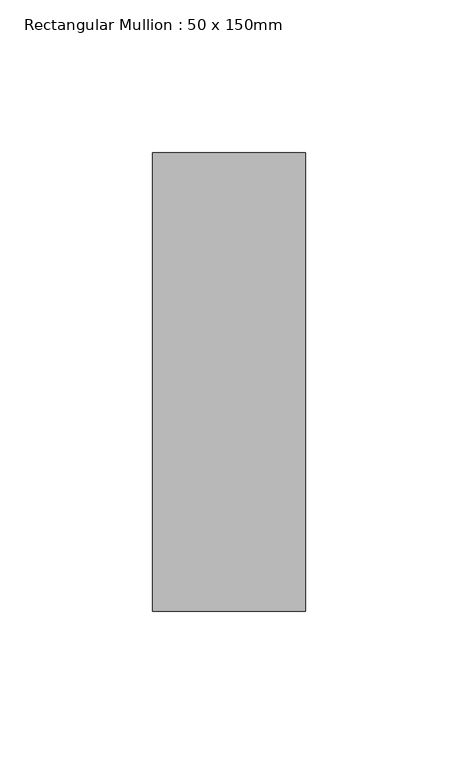
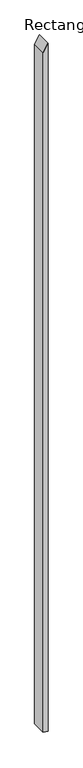
"""IFC4 building model written with IfcOpenShell, lengths in millimetres: member geometry, Rectangular Mullion : 50 x 150mm."""

import ifcopenshell
import ifcopenshell.guid

model = None  # the IFC model being written
_history = None  # IfcOwnerHistory: only IFC2X3 demands one
_inside = {}  # id of a spatial element -> (the spatial element, [elements in it])
_under = {}  # id of a project, library or spatial element -> (it, [spatial elements below it])
_declared = {}  # id of a project -> (the project, [libraries it declares])
_typed = {}  # id of a type object -> (the type object, [elements of that type])
_made_of = {}  # id of a material, layer set ... -> (it, [elements and type objects made of it])


def new_model(schema):
    """Start an empty IFC model of exactly this schema.

    Asked for "IFC4X3", IfcOpenShell would pick the latest addendum, in which some entities
    have other attributes; the version numbers below select the first issue.
    IFC2X3 requires an IfcOwnerHistory on every rooted entity: one is made here for all.
    """
    global model, _history
    if schema == "IFC4X3":
        model = ifcopenshell.file(schema_version=(4, 3, 0, 0))
    else:
        model = ifcopenshell.file(schema=schema)
    _inside.clear()
    _under.clear()
    _declared.clear()
    _typed.clear()
    _made_of.clear()
    _history = None
    if model.schema == "IFC2X3":
        org = make("IfcOrganization", Name="unknown")
        user = make(
            "IfcPersonAndOrganization",
            ThePerson=make("IfcPerson", FamilyName="unknown"),
            TheOrganization=org,
        )
        app = make(
            "IfcApplication",
            ApplicationDeveloper=org,
            Version="unknown",
            ApplicationFullName="unknown",
            ApplicationIdentifier="unknown",
        )
        _history = make(
            "IfcOwnerHistory",
            OwningUser=user,
            OwningApplication=app,
            ChangeAction="ADDED",
            CreationDate=0,
        )
    return model


def make(cls, **values):
    """One entity of the class cls with the attributes given. An attribute that is None is left unset."""
    return model.create_entity(
        cls, **{name: value for name, value in values.items() if value is not None}
    )


def rooted(cls, **values):
    """An entity with a GlobalId (a new one), such as an element, a storey or a relation."""
    return make(cls, GlobalId=ifcopenshell.guid.new(), OwnerHistory=_history, **values)


def si_unit(unit_type, name, prefix=None):
    """IfcSIUnit, for example si_unit("LENGTHUNIT", "METRE", prefix="MILLI")."""
    return make("IfcSIUnit", UnitType=unit_type, Prefix=prefix, Name=name)


def assignment(units):
    """IfcUnitAssignment: the units of a project."""
    return None if units is None else make("IfcUnitAssignment", Units=units)


def point(xyz):
    """IfcCartesianPoint."""
    return None if xyz is None else make("IfcCartesianPoint", Coordinates=xyz)


def direction(xyz):
    """IfcDirection."""
    return None if xyz is None else make("IfcDirection", DirectionRatios=xyz)


def frame(location, z_axis=None, x_axis=None):
    """IfcAxis2Placement3D, a coordinate frame: its origin and axes. An axis left out is left unset."""
    return make(
        "IfcAxis2Placement3D",
        Location=point(location),
        Axis=direction(z_axis),
        RefDirection=direction(x_axis),
    )


def origin():
    """The frame at (0, 0, 0) with its axes left unset."""
    return frame((0.0, 0.0, 0.0))


def place(relative_to, where):
    """IfcLocalPlacement: puts the frame where relative to a parent placement (None: the world)."""
    return make(
        "IfcLocalPlacement", PlacementRelTo=relative_to, RelativePlacement=where
    )


def context(
    kind, dimensions, precision=None, world=None, true_north=None, identifier=None
):
    """IfcGeometricRepresentationContext, for example the 3D "Model" context."""
    return make(
        "IfcGeometricRepresentationContext",
        ContextIdentifier=identifier,
        ContextType=kind,
        CoordinateSpaceDimension=dimensions,
        Precision=precision,
        WorldCoordinateSystem=world,
        TrueNorth=true_north,
    )


def project(units=None, contexts=None):
    """IfcProject with its units and contexts."""
    return rooted(
        "IfcProject",
        Name="project",
        RepresentationContexts=contexts,
        UnitsInContext=assignment(units),
    )


def spatial(cls, under=None, at=None, **own):
    """A site, building, storey or space (cls), placed at a placement, below another one or the project."""
    s = rooted(cls, ObjectPlacement=at, **own)
    if under is not None:
        _under.setdefault(under.id(), (under, []))[1].append(s)
    return s


def polyline(points):
    """IfcPolyline through the points."""
    return make("IfcPolyline", Points=[point(p) for p in points])


def outline(outer, holes=None, kind="AREA"):
    """IfcArbitraryClosedProfileDef: a profile drawn as a closed curve; with holes, ...WithVoids."""
    if holes is None:
        return make("IfcArbitraryClosedProfileDef", ProfileType=kind, OuterCurve=outer)
    return make(
        "IfcArbitraryProfileDefWithVoids",
        ProfileType=kind,
        OuterCurve=outer,
        InnerCurves=holes,
    )


def extrude(swept, where, along, depth):
    """IfcExtrudedAreaSolid: the profile swept, set in the frame where, extruded along a direction by depth."""
    return make(
        "IfcExtrudedAreaSolid",
        SweptArea=swept,
        Position=where,
        ExtrudedDirection=direction(along),
        Depth=depth,
    )


def shape(context_of_items, identifier, shape_type, items):
    """IfcShapeRepresentation: the items that make up one representation, for example the "Body"."""
    return make(
        "IfcShapeRepresentation",
        ContextOfItems=context_of_items,
        RepresentationIdentifier=identifier,
        RepresentationType=shape_type,
        Items=items,
    )


def source(mapping_origin, context_of_items, identifier, shape_type, items):
    """IfcRepresentationMap: a shape defined once, which mapped items show again and again."""
    return make(
        "IfcRepresentationMap",
        MappingOrigin=mapping_origin,
        MappedRepresentation=shape(context_of_items, identifier, shape_type, items),
    )


def transform(
    local_origin,
    x_axis=None,
    y_axis=None,
    z_axis=None,
    scale=None,
    scale2=None,
    scale3=None,
    uniform=True,
):
    """IfcCartesianTransformationOperator3D, or its non-uniform kind. x_axis, y_axis, z_axis: its Axis1, 2, 3."""
    if uniform:
        return make(
            "IfcCartesianTransformationOperator3D",
            Axis1=direction(x_axis),
            Axis2=direction(y_axis),
            LocalOrigin=point(local_origin),
            Scale=scale,
            Axis3=direction(z_axis),
        )
    return make(
        "IfcCartesianTransformationOperator3DnonUniform",
        Axis1=direction(x_axis),
        Axis2=direction(y_axis),
        LocalOrigin=point(local_origin),
        Scale=scale,
        Axis3=direction(z_axis),
        Scale2=scale2,
        Scale3=scale3,
    )


def mapped(mapping_source, mapping_target):
    """IfcMappedItem: shows the shape of a source again, moved by a transform."""
    return make(
        "IfcMappedItem", MappingSource=mapping_source, MappingTarget=mapping_target
    )


def made_of(thing, what):
    """Note that an element or type object is made of a material, layer set ...; save() writes the relation."""
    if what is not None:
        _made_of.setdefault(what.id(), (what, []))[1].append(thing)
    return thing


def element(
    cls,
    number,
    at=None,
    inside=None,
    cuts=None,
    type_object=None,
    material=None,
    context=None,
    identifier="Body",
    shape_type=None,
    held_by="IfcProductDefinitionShape",
    body=None,
    shapes=None,
    **own,
):
    """One element of the class cls, such as IfcWall. Its Tag is "e" and its number.

    at: its placement. inside: the storey or other place that contains it. cuts: it is an
    opening in that element (IfcRelVoidsElement). A single representation is given by context,
    identifier, shape_type and body (its items); several are given by shapes. held_by: the class
    of the entity that holds the representations. save() writes the other relations.
    """
    e = rooted(cls, Tag="e%d" % number, ObjectPlacement=at, **own)
    if body is not None:
        shapes = [shape(context, identifier, shape_type, body)]
    if shapes is not None:
        e.Representation = make(held_by, Representations=shapes)
    if inside is not None:
        _inside.setdefault(inside.id(), (inside, []))[1].append(e)
    if cuts is not None:
        rooted(
            "IfcRelVoidsElement", RelatingBuildingElement=cuts, RelatedOpeningElement=e
        )
    if type_object is not None:
        _typed.setdefault(type_object.id(), (type_object, []))[1].append(e)
    return made_of(e, material)


def aggregate(whole, parts):
    """IfcRelAggregates: a whole, such as a stair, and the parts it consists of."""
    return rooted("IfcRelAggregates", RelatingObject=whole, RelatedObjects=parts)


def save(model, path):
    """Write the relations noted so far, then the file.

    IfcRelAggregates (storeys below a building ...), IfcRelContainedInSpatialStructure (elements
    in a storey), IfcRelDefinesByType, IfcRelAssociatesMaterial and IfcRelDeclares: one each for
    every whole, place, type object, material and project.
    """
    for whole, parts in _under.values():
        aggregate(whole, parts)
    for where, things in _inside.values():
        rooted(
            "IfcRelContainedInSpatialStructure",
            RelatedElements=things,
            RelatingStructure=where,
        )
    for kind, things in _typed.values():
        rooted("IfcRelDefinesByType", RelatedObjects=things, RelatingType=kind)
    for what, things in _made_of.values():
        rooted("IfcRelAssociatesMaterial", RelatedObjects=things, RelatingMaterial=what)
    for by, libraries in _declared.values():
        rooted("IfcRelDeclares", RelatingContext=by, RelatedDefinitions=libraries)
    model.write(path)


def rectangular_mullion_50_x_150mm_7805e086(model_context):
    return source(origin(), model_context, "Body", "SweptSolid", [
        extrude(outline(polyline([(0.0, 0.0), (-85.321119, -50.0), (-7488.5336568, -50.0), (-7500.253691, 0.0), (0.0, 0.0)])), frame((0.0, -75.0, 0.0), z_axis=(0.0, 1.0, 0.0), x_axis=(0.0, 0.0, 1.0)), (0.0, 0.0, 1.0), 150.0),
    ])


if __name__ == "__main__":
    model = new_model("IFC4")
    model_context = context("Model", 3, world=origin())
    ifc_project = project(units=[si_unit("LENGTHUNIT", "METRE", prefix="MILLI")], contexts=[model_context])
    site = spatial("IfcSite", under=ifc_project)
    building = spatial("IfcBuilding", under=site)
    placement = place(None, origin())
    rectangular_mullion_50_x_150mm_shape = rectangular_mullion_50_x_150mm_7805e086(model_context)
    element("IfcMember", 1, ObjectType="Rectangular Mullion : 50 x 150mm", at=placement, inside=building, context=model_context, shape_type="MappedRepresentation", body=[
        mapped(rectangular_mullion_50_x_150mm_shape, transform((0.0, 0.0, 0.0), x_axis=(1.0, 0.0, 0.0), y_axis=(0.0, 1.0, 0.0), z_axis=(0.0, 0.0, 1.0))),
    ])
    save(model, "model.ifc")

# Revit data of these elements
# Type "Rectangular Mullion : 50 x 150mm"
#   built-in parameter 1007304 = 0.492126 (stored number, unit not read)
#   built-in parameter 1007301 = 0.082021 (stored number, unit not read)
#   built-in parameter 1007300 = 0.082021 (stored number, unit not read)
# Element 1 (IfcMember, "Rectangular Mullion : 50 x 150mm")
#   Materials on its faces: "Metal - Aluminium"
# Materials
#   "Metal - Aluminium": class "Metal", colour RGB 247 247 247, transparency 0
